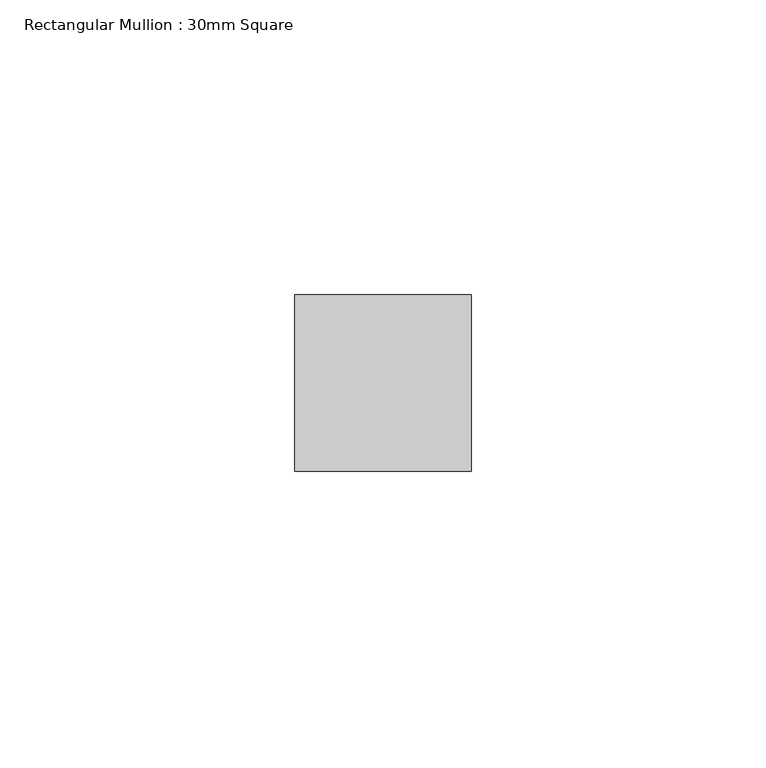
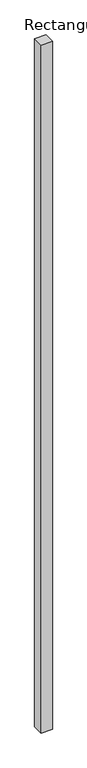
"""IFC4 building model written with IfcOpenShell, lengths in millimetres: member geometry, Rectangular Mullion : 30mm Square."""

from ifc_helpers import new_model, si_unit, frame, origin, place, context, project, spatial, polyline, outline, extrude, source, transform, mapped, element, save


def rectangular_mullion_30mm_square_1bad5264(model_context):
    return source(origin(), model_context, "Body", "SweptSolid", [
        extrude(outline(polyline([(15.0, 15.0), (15.0, -15.0), (-15.0, -15.0), (-15.0, 15.0), (15.0, 15.0)])), frame((0.0, 0.0, -1947.739401), z_axis=(0.0, 0.0, 1.0), x_axis=(1.0, 0.0, 0.0)), (0.0, 0.0, 1.0), 1947.739401),
    ])


if __name__ == "__main__":
    model = new_model("IFC4")
    model_context = context("Model", 3, world=origin())
    ifc_project = project(units=[si_unit("LENGTHUNIT", "METRE", prefix="MILLI")], contexts=[model_context])
    site = spatial("IfcSite", under=ifc_project)
    building = spatial("IfcBuilding", under=site)
    placement = place(None, origin())
    rectangular_mullion_30mm_square_shape = rectangular_mullion_30mm_square_1bad5264(model_context)
    element("IfcMember", 1, ObjectType="Rectangular Mullion : 30mm Square", at=placement, inside=building, context=model_context, shape_type="MappedRepresentation", body=[
        mapped(rectangular_mullion_30mm_square_shape, transform((0.0, 0.0, 0.0), x_axis=(1.0, 0.0, 0.0), y_axis=(0.0, 1.0, 0.0), z_axis=(0.0, 0.0, 1.0))),
    ])
    save(model, "model.ifc")

# Revit data of these elements
# Type "Rectangular Mullion : 30mm Square"
#   built-in parameter 1007304 = 0.0984252 (stored number, unit not read)
#   built-in parameter 1007301 = 0.0492126 (stored number, unit not read)
#   built-in parameter 1007300 = 0.0492126 (stored number, unit not read)
# Element 1 (IfcMember, "Rectangular Mullion : 30mm Square")
#   Materials on its faces: "Aluminum"
# Materials
#   "Aluminum": class "Metal", colour RGB 244 244 244, transparency 0, Description = "Aluminum 6061", Cost = 0
